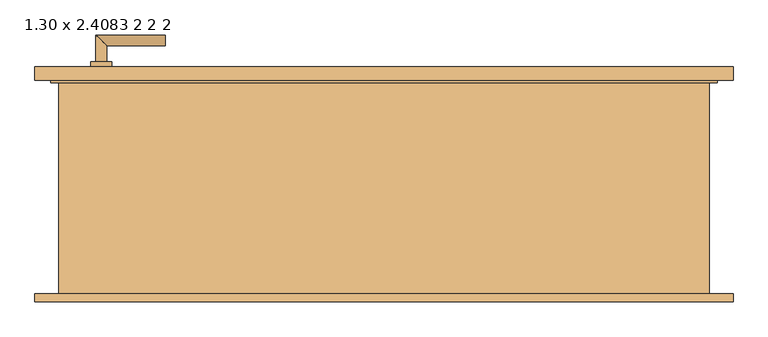
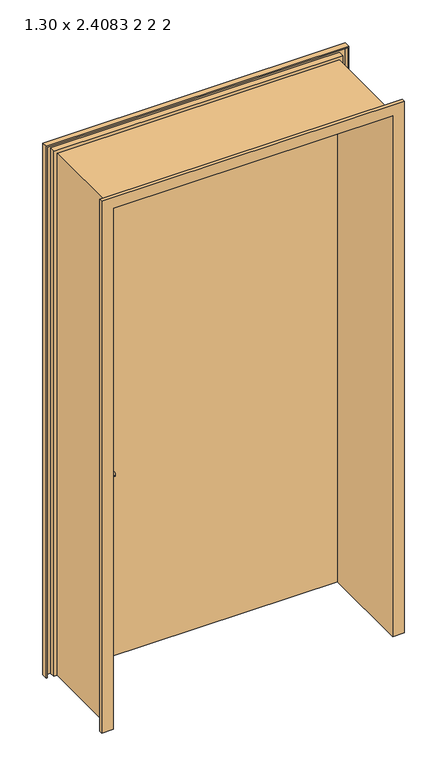
"""IFC4 building model written with IfcOpenShell, lengths in millimetres: door geometry, Drehflügel 1-flg - Stahlzarge : 1.30 x 2.4083 2 2 2."""

from ifc_helpers import new_model, si_unit, point, frame, frame_2d, origin, place, context, project, spatial, polyline, circle_curve, ellipse_curve, trimmed, segment, composite_curve, outline, extrude, faceted_brep, source, transform, mapped, element, save
from ifc_brep_helpers import plane_surface, cylinder_surface, advanced_brep


def door_1_30_x_2_4083_2_2_2_c68c049b(model_context):
    return source(origin(), model_context, "Body", "SolidModel", [
        advanced_brep(
        [(-540.0, 189.4346141, 915.0), (-520.0, 189.4346141, 915.0), (-540.0, 119.4346141, 915.0), (-520.0, 139.4346141, 915.0), (-410.0, 119.4346141, 915.0), (-410.0, 139.4346141, 915.0)],
        [
            (0, 1, circle_curve(frame((-530.0, 189.4346141, 915.0), z_axis=(0.0, 1.0, 0.0), x_axis=(1.0, 0.0, 0.0)), 10.0)),
            (1, 0, circle_curve(frame((-530.0, 189.4346141, 915.0), z_axis=(0.0, 1.0, 0.0), x_axis=(1.0, 0.0, 0.0)), 10.0)),
            (0, 2),
            (2, 3, ellipse_curve(frame((-530.0, 129.4346141, 915.0), z_axis=(-0.7071067811865385, 0.7071067811865565, 0.0), x_axis=(0.7071067811865563, 0.7071067811865386, 0.0)), 14.1421356, 10.0)),
            (3, 1),
            (3, 2, ellipse_curve(frame((-530.0, 129.4346141, 915.0), z_axis=(-0.7071067811865385, 0.7071067811865565, 0.0), x_axis=(0.7071067811865563, 0.7071067811865386, 0.0)), 14.1421356, 10.0)),
            (4, 5, circle_curve(frame((-410.0, 129.4346141, 915.0), z_axis=(1.0, 0.0, 0.0), x_axis=(0.0, 1.0, 0.0)), 10.0)),
            (5, 4, circle_curve(frame((-410.0, 129.4346141, 915.0), z_axis=(1.0, 0.0, 0.0), x_axis=(0.0, 1.0, 0.0)), 10.0)),
            (2, 4),
            (5, 3),
        ],
        [
            plane_surface(frame((-530.0, 189.4346141, -372.7526403), z_axis=(0.0, 1.0, 0.0), x_axis=(0.0, 0.0, 1.0))),
            cylinder_surface(frame((-530.0, 189.4346141, 915.0), z_axis=(0.0, 1.0, 0.0), x_axis=(1.0, 0.0, 0.0)), 10.0),
            plane_surface(frame((-410.0, 129.4346141, -372.7526403), z_axis=(1.0, 0.0, 0.0), x_axis=(0.0, 0.0, 1.0))),
            cylinder_surface(frame((-530.0, 129.4346141, 915.0), z_axis=(-1.0, 0.0, 0.0), x_axis=(0.0, 1.0, 0.0)), 10.0),
        ],
        [
            (0, [[1, 2]]),
            (1, [[-1, 3, 4, 5]]),
            (1, [[-2, -5, 6, -3]]),
            (2, [[7, 8]]),
            (3, [[-4, 9, -8, 10]]),
            (3, [[-6, -10, -7, -9]]),
        ],
    ),
        advanced_brep(
        [(-520.0, 249.4346141, 915.0), (-540.0, 249.4346141, 915.0), (-520.0, 279.4346141, 915.0), (-540.0, 299.4346141, 915.0), (-410.0, 279.4346141, 915.0), (-410.0, 299.4346141, 915.0)],
        [
            (0, 1, circle_curve(frame((-530.0, 249.4346141, 915.0), z_axis=(0.0, -1.0, 0.0), x_axis=(-1.0, 0.0, 0.0)), 10.0)),
            (1, 0, circle_curve(frame((-530.0, 249.4346141, 915.0), z_axis=(0.0, -1.0, 0.0), x_axis=(-1.0, 0.0, 0.0)), 10.0)),
            (0, 2),
            (2, 3, ellipse_curve(frame((-530.0, 289.4346141, 915.0), z_axis=(-0.7071067811865475, -0.7071067811865475, 0.0), x_axis=(0.7071067811865474, -0.7071067811865476, 0.0)), 14.1421356, 10.0)),
            (3, 1),
            (3, 2, ellipse_curve(frame((-530.0, 289.4346141, 915.0), z_axis=(-0.7071067811865475, -0.7071067811865475, 0.0), x_axis=(0.7071067811865474, -0.7071067811865476, 0.0)), 14.1421356, 10.0)),
            (4, 5, circle_curve(frame((-410.0, 289.4346141, 915.0), z_axis=(1.0, 0.0, 0.0), x_axis=(0.0, 1.0, 0.0)), 10.0)),
            (5, 4, circle_curve(frame((-410.0, 289.4346141, 915.0), z_axis=(1.0, 0.0, 0.0), x_axis=(0.0, 1.0, 0.0)), 10.0)),
            (2, 4),
            (5, 3),
        ],
        [
            plane_surface(frame((-530.0, 249.4346141, -372.7526403), z_axis=(0.0, -1.0, 0.0), x_axis=(0.0, 0.0, 1.0))),
            cylinder_surface(frame((-530.0, 249.4346141, 915.0), z_axis=(0.0, -1.0, 0.0), x_axis=(-1.0, 0.0, 0.0)), 10.0),
            plane_surface(frame((-410.0, 289.4346141, -372.7526403), z_axis=(1.0, 0.0, 0.0), x_axis=(0.0, 0.0, 1.0))),
            cylinder_surface(frame((-530.0, 289.4346141, 915.0), z_axis=(-1.0, 0.0, 0.0), x_axis=(0.0, 1.0, 0.0)), 10.0),
        ],
        [
            (0, [[1, 2]]),
            (1, [[-1, 3, 4, 5]]),
            (1, [[-2, -5, 6, -3]]),
            (2, [[7, 8]]),
            (3, [[-4, 9, -8, 10]]),
            (3, [[-6, -10, -7, -9]]),
        ],
    ),
        extrude(outline(composite_curve([segment(trimmed(circle_curve(frame_2d((915.0, -530.0)), 20.0), [point((915.0, -550.0))], [point((915.0, -510.0))], False, "CARTESIAN"), True, "CONTINUOUS"), segment(trimmed(circle_curve(frame_2d((915.0, -530.0)), 20.0), [point((915.0, -510.0))], [point((915.0, -550.0))], False, "CARTESIAN"), True, "CONTINUOUS")], self_intersect=False)), frame((0.0, 179.4346141, 0.0), z_axis=(0.0, 1.0, 0.0), x_axis=(0.0, 0.0, 1.0)), (0.0, 0.0, 1.0), 10.0),
        extrude(outline(composite_curve([segment(trimmed(circle_curve(frame_2d((915.0, -530.0)), 20.0), [point((915.0, -550.0))], [point((915.0, -510.0))], False, "CARTESIAN"), True, "CONTINUOUS"), segment(trimmed(circle_curve(frame_2d((915.0, -530.0)), 20.0), [point((915.0, -510.0))], [point((915.0, -550.0))], False, "CARTESIAN"), True, "CONTINUOUS")], self_intersect=False)), frame((0.0, 239.4346141, 0.0), z_axis=(0.0, 1.0, 0.0), x_axis=(0.0, 0.0, 1.0)), (0.0, 0.0, 1.0), 10.0),
        extrude(outline(polyline([(620.0, 214.4346141), (-620.0, 214.4346141), (-620.0, 239.4346141), (620.0, 239.4346141), (620.0, 214.4346141)])), frame((0.0, 0.0, 15.0), z_axis=(0.0, 0.0, 1.0), x_axis=(1.0, 0.0, 0.0)), (0.0, 0.0, 1.0), 2398.3),
        faceted_brep([(654.4603207, -200.5653859, 15.0), (605.0, -200.5653859, 15.0), (605.0, 214.4346141, 15.0), (620.0, 214.4346141, 15.0), (620.0, 239.4346141, 15.0), (654.4603207, 239.4346141, 15.0), (654.4603207, 214.4346141, 15.0), (649.4603207, 214.4346141, 15.0), (649.4603207, 234.4346141, 15.0), (625.0, 234.4346141, 15.0), (625.0, 209.4346141, 15.0), (610.0, 209.4346141, 15.0), (610.0, -195.5653859, 15.0), (649.4603207, -195.5653859, 15.0), (649.4603207, -185.5653859, 15.0), (654.4603207, -185.5653859, 15.0), (654.4603207, -200.5653859, 2447.7603207), (-654.4603207, -200.5653859, 2447.7603207), (-654.4603207, -200.5653859, 15.0), (-605.0, -200.5653859, 15.0), (-605.0, -200.5653859, 2398.3), (605.0, -200.5653859, 2398.3), (605.0, 214.4346141, 2398.3), (-605.0, 214.4346141, 2398.3), (-605.0, 214.4346141, 15.0), (-620.0, 214.4346141, 15.0), (-620.0, 214.4346141, 2413.3), (620.0, 214.4346141, 2413.3), (620.0, 239.4346141, 2413.3), (-620.0, 239.4346141, 2413.3), (-620.0, 239.4346141, 15.0), (-654.4603207, 239.4346141, 15.0), (-654.4603207, 239.4346141, 2447.7603207), (654.4603207, 239.4346141, 2447.7603207), (654.4603207, 214.4346141, 2447.7603207), (-654.4603207, 214.4346141, 2447.7603207), (-654.4603207, 214.4346141, 15.0), (-649.4603207, 214.4346141, 15.0), (-649.4603207, 214.4346141, 2442.7603207), (649.4603207, 214.4346141, 2442.7603207), (649.4603207, 234.4346141, 2442.7603207), (-649.4603207, 234.4346141, 2442.7603207), (-649.4603207, 234.4346141, 15.0), (-625.0, 234.4346141, 15.0), (-625.0, 234.4346141, 2418.3), (625.0, 234.4346141, 2418.3), (625.0, 209.4346141, 2418.3), (-625.0, 209.4346141, 2418.3), (-625.0, 209.4346141, 15.0), (-610.0, 209.4346141, 15.0), (-610.0, 209.4346141, 2403.3), (610.0, 209.4346141, 2403.3), (610.0, -195.5653859, 2403.3), (-610.0, -195.5653859, 2403.3), (-610.0, -195.5653859, 15.0), (-649.4603207, -195.5653859, 15.0), (-649.4603207, -195.5653859, 2442.7603207), (649.4603207, -195.5653859, 2442.7603207), (649.4603207, -185.5653859, 2442.7603207), (-649.4603207, -185.5653859, 2442.7603207), (-649.4603207, -185.5653859, 15.0), (-654.4603207, -185.5653859, 15.0), (-654.4603207, -185.5653859, 2447.7603207), (654.4603207, -185.5653859, 2447.7603207)], [[[0, 1, 2, 3, 4, 5, 6, 7, 8, 9, 10, 11, 12, 13, 14, 15]], [[1, 0, 16, 17, 18, 19, 20, 21]], [[2, 1, 21, 22]], [[3, 2, 22, 23, 24, 25, 26, 27]], [[4, 3, 27, 28]], [[5, 4, 28, 29, 30, 31, 32, 33]], [[6, 5, 33, 34]], [[7, 6, 34, 35, 36, 37, 38, 39]], [[8, 7, 39, 40]], [[9, 8, 40, 41, 42, 43, 44, 45]], [[10, 9, 45, 46]], [[11, 10, 46, 47, 48, 49, 50, 51]], [[12, 11, 51, 52]], [[13, 12, 52, 53, 54, 55, 56, 57]], [[14, 13, 57, 58]], [[15, 14, 58, 59, 60, 61, 62, 63]], [[0, 15, 63, 16]], [[17, 62, 61, 18]], [[18, 61, 60, 55, 54, 49, 48, 43, 42, 37, 36, 31, 30, 25, 24, 19]], [[23, 20, 19, 24]], [[29, 26, 25, 30]], [[35, 32, 31, 36]], [[41, 38, 37, 42]], [[47, 44, 43, 48]], [[53, 50, 49, 54]], [[59, 56, 55, 60]], [[22, 21, 20, 23]], [[28, 27, 26, 29]], [[34, 33, 32, 35]], [[40, 39, 38, 41]], [[46, 45, 44, 47]], [[52, 51, 50, 53]], [[58, 57, 56, 59]], [[16, 63, 62, 17]]]),
    ])


if __name__ == "__main__":
    model = new_model("IFC4")
    model_context = context("Model", 3, world=origin())
    ifc_project = project(units=[si_unit("LENGTHUNIT", "METRE", prefix="MILLI")], contexts=[model_context])
    site = spatial("IfcSite", under=ifc_project)
    building = spatial("IfcBuilding", under=site)
    placement = place(None, origin())
    door_1_30_x_2_4083_2_2_2_shape = door_1_30_x_2_4083_2_2_2_c68c049b(model_context)
    element("IfcDoor", 1, ObjectType="Drehflügel 1-flg - Stahlzarge : 1.30 x 2.4083 2 2 2", at=placement, inside=building, context=model_context, shape_type="MappedRepresentation", body=[
        mapped(door_1_30_x_2_4083_2_2_2_shape, transform((0.0, 0.0, 0.0), x_axis=(1.0, 0.0, 0.0), y_axis=(0.0, 1.0, 0.0), z_axis=(0.0, 0.0, 1.0))),
    ])
    save(model, "model.ifc")

# Revit data of these elements
# Type "Drehflügel 1-flg - Stahlzarge : 1.30 x 2.4083 2 2 2"
#   Type Mark = "26"
#   Operation = "SingleSwingRight"
#   Keynote = "16.03"
#   Analytic Construction = "Metall"
#   Thermal Resistance (R) = 0.270117 (m²·K)/W
#   Heat Transfer Coefficient (U) = 3.7021 W/(m²·K)
#   Rough Width = 1.260 m
#   Rough Height [instance default] = 2.5083 m
#   Höhe Türgriff [instance default] = 0.900 m
#   Height = 2.4083 m
#   Fußbodenaufbau [instance default] = 0.100 m
#   Width = 1.260 m
#   Sichtbarkeit Sturzlinien [instance default] = yes
#   Türgriff auswählen [instance default] = element 221079
#   Türgriff [instance default] = none
#   Türflügel [instance default] = none
#   Rahmen/Pfosten [instance default] = Metall - Lackiert - Grau
#   Visual Light Transmittance = 0
#   Solar Heat Gain Coefficient = 0
#   Function = (empty or 0)
#   Wall Closure = (empty or 0)
# Element 1 (IfcDoor, "Drehflügel 1-flg - Stahlzarge : 1.30 x 2.4083 2 2 2")
#   Rough Height = 2.4233 m
#   Fußbodenaufbau = 0.015 m
#   Materials on its faces: "Metall - Lackiert - Grau", "Metall - Chrom", "Holz - Birke"
# Materials
#   "Metall - Lackiert - Grau": class "Farbe 1", colour RGB 98 98 98, transparency 0, Cost = 0
#   "Metall - Chrom": class "Metall", colour RGB 247 247 247, transparency 0, Cost = 0
#   "Holz - Birke": class "Holz", colour RGB 213 164 103, transparency 0, Cost = 0
